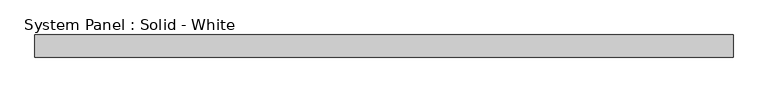
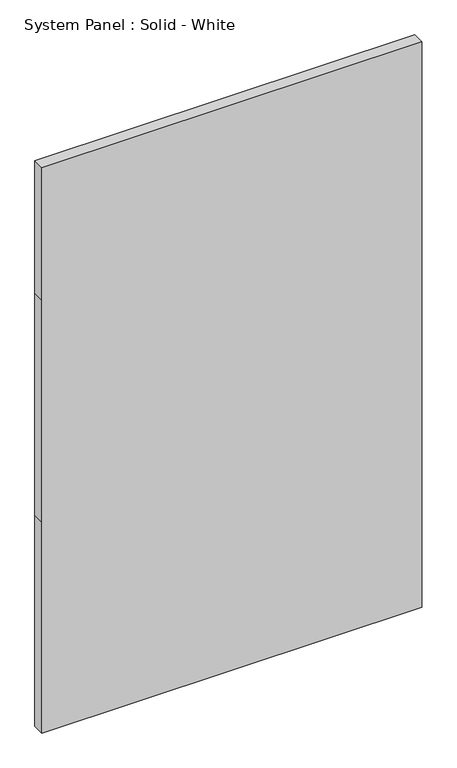
"""IFC4 building model written with IfcOpenShell, lengths in millimetres: plate geometry, System Panel : Solid - White."""

from ifc_helpers import new_model, si_unit, frame, origin, place, context, project, spatial, polyline, outline, extrude, source, transform, mapped, element, save


def system_panel_solid_white_b427edf1(model_context):
    return source(origin(), model_context, "Body", "SweptSolid", [
        extrude(outline(polyline([(0.0, -985.4757062), (0.0, 985.4757062), (1155.7, 985.4757062), (2374.9, 985.4757062), (3101.9419949, 985.4757062), (3101.9419949, -985.4757062), (2374.9, -985.4757062), (1155.7, -985.4757062), (0.0, -985.4757062)])), frame((0.0, -44.45, 0.0), z_axis=(0.0, 1.0, 0.0), x_axis=(0.0, 0.0, 1.0)), (0.0, 0.0, 1.0), 63.5),
    ])


if __name__ == "__main__":
    model = new_model("IFC4")
    model_context = context("Model", 3, world=origin())
    ifc_project = project(units=[si_unit("LENGTHUNIT", "METRE", prefix="MILLI")], contexts=[model_context])
    site = spatial("IfcSite", under=ifc_project)
    building = spatial("IfcBuilding", under=site)
    placement = place(None, origin())
    system_panel_solid_white_shape = system_panel_solid_white_b427edf1(model_context)
    element("IfcPlate", 1, ObjectType="System Panel : Solid - White", at=placement, inside=building, context=model_context, shape_type="MappedRepresentation", body=[
        mapped(system_panel_solid_white_shape, transform((0.0, 0.0, 0.0), x_axis=(1.0, 0.0, 0.0), y_axis=(0.0, 1.0, 0.0), z_axis=(0.0, 0.0, 1.0))),
    ])
    save(model, "model.ifc")

# Revit data of these elements
# Element 1 (IfcPlate, "System Panel : Solid - White")
#   Materials on its faces: "White Panel"
# Materials
#   "White Panel": class "Unassigned", colour RGB 255 255 255, transparency 0
